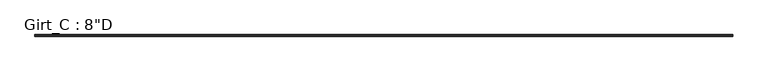
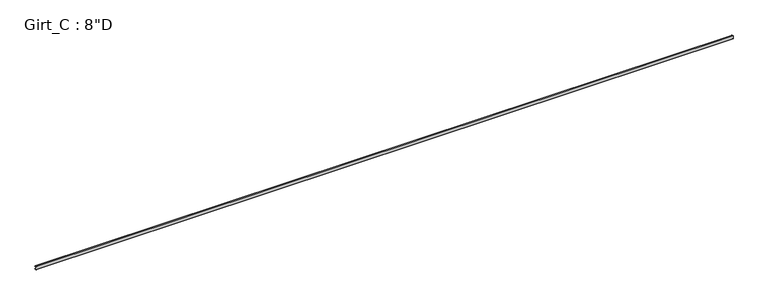
"""IFC4 building model written with IfcOpenShell, lengths in millimetres: beam geometry."""

import ifcopenshell
import ifcopenshell.guid

model = None  # the IFC model being written
_history = None  # IfcOwnerHistory: only IFC2X3 demands one
_inside = {}  # id of a spatial element -> (the spatial element, [elements in it])
_under = {}  # id of a project, library or spatial element -> (it, [spatial elements below it])
_declared = {}  # id of a project -> (the project, [libraries it declares])
_typed = {}  # id of a type object -> (the type object, [elements of that type])
_made_of = {}  # id of a material, layer set ... -> (it, [elements and type objects made of it])


def new_model(schema):
    """Start an empty IFC model of exactly this schema.

    Asked for "IFC4X3", IfcOpenShell would pick the latest addendum, in which some entities
    have other attributes; the version numbers below select the first issue.
    IFC2X3 requires an IfcOwnerHistory on every rooted entity: one is made here for all.
    """
    global model, _history
    if schema == "IFC4X3":
        model = ifcopenshell.file(schema_version=(4, 3, 0, 0))
    else:
        model = ifcopenshell.file(schema=schema)
    _inside.clear()
    _under.clear()
    _declared.clear()
    _typed.clear()
    _made_of.clear()
    _history = None
    if model.schema == "IFC2X3":
        org = make("IfcOrganization", Name="unknown")
        user = make(
            "IfcPersonAndOrganization",
            ThePerson=make("IfcPerson", FamilyName="unknown"),
            TheOrganization=org,
        )
        app = make(
            "IfcApplication",
            ApplicationDeveloper=org,
            Version="unknown",
            ApplicationFullName="unknown",
            ApplicationIdentifier="unknown",
        )
        _history = make(
            "IfcOwnerHistory",
            OwningUser=user,
            OwningApplication=app,
            ChangeAction="ADDED",
            CreationDate=0,
        )
    return model


def make(cls, **values):
    """One entity of the class cls with the attributes given. An attribute that is None is left unset."""
    return model.create_entity(
        cls, **{name: value for name, value in values.items() if value is not None}
    )


def rooted(cls, **values):
    """An entity with a GlobalId (a new one), such as an element, a storey or a relation."""
    return make(cls, GlobalId=ifcopenshell.guid.new(), OwnerHistory=_history, **values)


def si_unit(unit_type, name, prefix=None):
    """IfcSIUnit, for example si_unit("LENGTHUNIT", "METRE", prefix="MILLI")."""
    return make("IfcSIUnit", UnitType=unit_type, Prefix=prefix, Name=name)


def assignment(units):
    """IfcUnitAssignment: the units of a project."""
    return None if units is None else make("IfcUnitAssignment", Units=units)


def point(xyz):
    """IfcCartesianPoint."""
    return None if xyz is None else make("IfcCartesianPoint", Coordinates=xyz)


def direction(xyz):
    """IfcDirection."""
    return None if xyz is None else make("IfcDirection", DirectionRatios=xyz)


def frame(location, z_axis=None, x_axis=None):
    """IfcAxis2Placement3D, a coordinate frame: its origin and axes. An axis left out is left unset."""
    return make(
        "IfcAxis2Placement3D",
        Location=point(location),
        Axis=direction(z_axis),
        RefDirection=direction(x_axis),
    )


def frame_2d(location, x_axis=None):
    """IfcAxis2Placement2D, a coordinate frame in the plane: its origin and x axis."""
    return make(
        "IfcAxis2Placement2D", Location=point(location), RefDirection=direction(x_axis)
    )


def origin():
    """The frame at (0, 0, 0) with its axes left unset."""
    return frame((0.0, 0.0, 0.0))


def place(relative_to, where):
    """IfcLocalPlacement: puts the frame where relative to a parent placement (None: the world)."""
    return make(
        "IfcLocalPlacement", PlacementRelTo=relative_to, RelativePlacement=where
    )


def context(
    kind, dimensions, precision=None, world=None, true_north=None, identifier=None
):
    """IfcGeometricRepresentationContext, for example the 3D "Model" context."""
    return make(
        "IfcGeometricRepresentationContext",
        ContextIdentifier=identifier,
        ContextType=kind,
        CoordinateSpaceDimension=dimensions,
        Precision=precision,
        WorldCoordinateSystem=world,
        TrueNorth=true_north,
    )


def project(units=None, contexts=None):
    """IfcProject with its units and contexts."""
    return rooted(
        "IfcProject",
        Name="project",
        RepresentationContexts=contexts,
        UnitsInContext=assignment(units),
    )


def spatial(cls, under=None, at=None, **own):
    """A site, building, storey or space (cls), placed at a placement, below another one or the project."""
    s = rooted(cls, ObjectPlacement=at, **own)
    if under is not None:
        _under.setdefault(under.id(), (under, []))[1].append(s)
    return s


def polyline(points):
    """IfcPolyline through the points."""
    return make("IfcPolyline", Points=[point(p) for p in points])


def circle_curve(where, radius):
    """IfcCircle in the frame where."""
    return make("IfcCircle", Position=where, Radius=radius)


def trimmed(basis, trim1, trim2, sense, master):
    """IfcTrimmedCurve: the piece of a basis curve between two trims."""
    return make(
        "IfcTrimmedCurve",
        BasisCurve=basis,
        Trim1=trim1,
        Trim2=trim2,
        SenseAgreement=sense,
        MasterRepresentation=master,
    )


def segment(curve, same_sense, transition):
    """IfcCompositeCurveSegment."""
    return make(
        "IfcCompositeCurveSegment",
        Transition=transition,
        SameSense=same_sense,
        ParentCurve=curve,
    )


def composite_curve(segments, self_intersect=None):
    """IfcCompositeCurve: segments joined end to end."""
    return make("IfcCompositeCurve", Segments=segments, SelfIntersect=self_intersect)


def outline(outer, holes=None, kind="AREA"):
    """IfcArbitraryClosedProfileDef: a profile drawn as a closed curve; with holes, ...WithVoids."""
    if holes is None:
        return make("IfcArbitraryClosedProfileDef", ProfileType=kind, OuterCurve=outer)
    return make(
        "IfcArbitraryProfileDefWithVoids",
        ProfileType=kind,
        OuterCurve=outer,
        InnerCurves=holes,
    )


def extrude(swept, where, along, depth):
    """IfcExtrudedAreaSolid: the profile swept, set in the frame where, extruded along a direction by depth."""
    return make(
        "IfcExtrudedAreaSolid",
        SweptArea=swept,
        Position=where,
        ExtrudedDirection=direction(along),
        Depth=depth,
    )


def shape(context_of_items, identifier, shape_type, items):
    """IfcShapeRepresentation: the items that make up one representation, for example the "Body"."""
    return make(
        "IfcShapeRepresentation",
        ContextOfItems=context_of_items,
        RepresentationIdentifier=identifier,
        RepresentationType=shape_type,
        Items=items,
    )


def source(mapping_origin, context_of_items, identifier, shape_type, items):
    """IfcRepresentationMap: a shape defined once, which mapped items show again and again."""
    return make(
        "IfcRepresentationMap",
        MappingOrigin=mapping_origin,
        MappedRepresentation=shape(context_of_items, identifier, shape_type, items),
    )


def transform(
    local_origin,
    x_axis=None,
    y_axis=None,
    z_axis=None,
    scale=None,
    scale2=None,
    scale3=None,
    uniform=True,
):
    """IfcCartesianTransformationOperator3D, or its non-uniform kind. x_axis, y_axis, z_axis: its Axis1, 2, 3."""
    if uniform:
        return make(
            "IfcCartesianTransformationOperator3D",
            Axis1=direction(x_axis),
            Axis2=direction(y_axis),
            LocalOrigin=point(local_origin),
            Scale=scale,
            Axis3=direction(z_axis),
        )
    return make(
        "IfcCartesianTransformationOperator3DnonUniform",
        Axis1=direction(x_axis),
        Axis2=direction(y_axis),
        LocalOrigin=point(local_origin),
        Scale=scale,
        Axis3=direction(z_axis),
        Scale2=scale2,
        Scale3=scale3,
    )


def mapped(mapping_source, mapping_target):
    """IfcMappedItem: shows the shape of a source again, moved by a transform."""
    return make(
        "IfcMappedItem", MappingSource=mapping_source, MappingTarget=mapping_target
    )


def made_of(thing, what):
    """Note that an element or type object is made of a material, layer set ...; save() writes the relation."""
    if what is not None:
        _made_of.setdefault(what.id(), (what, []))[1].append(thing)
    return thing


def element(
    cls,
    number,
    at=None,
    inside=None,
    cuts=None,
    type_object=None,
    material=None,
    context=None,
    identifier="Body",
    shape_type=None,
    held_by="IfcProductDefinitionShape",
    body=None,
    shapes=None,
    **own,
):
    """One element of the class cls, such as IfcWall. Its Tag is "e" and its number.

    at: its placement. inside: the storey or other place that contains it. cuts: it is an
    opening in that element (IfcRelVoidsElement). A single representation is given by context,
    identifier, shape_type and body (its items); several are given by shapes. held_by: the class
    of the entity that holds the representations. save() writes the other relations.
    """
    e = rooted(cls, Tag="e%d" % number, ObjectPlacement=at, **own)
    if body is not None:
        shapes = [shape(context, identifier, shape_type, body)]
    if shapes is not None:
        e.Representation = make(held_by, Representations=shapes)
    if inside is not None:
        _inside.setdefault(inside.id(), (inside, []))[1].append(e)
    if cuts is not None:
        rooted(
            "IfcRelVoidsElement", RelatingBuildingElement=cuts, RelatedOpeningElement=e
        )
    if type_object is not None:
        _typed.setdefault(type_object.id(), (type_object, []))[1].append(e)
    return made_of(e, material)


def aggregate(whole, parts):
    """IfcRelAggregates: a whole, such as a stair, and the parts it consists of."""
    return rooted("IfcRelAggregates", RelatingObject=whole, RelatedObjects=parts)


def save(model, path):
    """Write the relations noted so far, then the file.

    IfcRelAggregates (storeys below a building ...), IfcRelContainedInSpatialStructure (elements
    in a storey), IfcRelDefinesByType, IfcRelAssociatesMaterial and IfcRelDeclares: one each for
    every whole, place, type object, material and project.
    """
    for whole, parts in _under.values():
        aggregate(whole, parts)
    for where, things in _inside.values():
        rooted(
            "IfcRelContainedInSpatialStructure",
            RelatedElements=things,
            RelatingStructure=where,
        )
    for kind, things in _typed.values():
        rooted("IfcRelDefinesByType", RelatedObjects=things, RelatingType=kind)
    for what, things in _made_of.values():
        rooted("IfcRelAssociatesMaterial", RelatedObjects=things, RelatingMaterial=what)
    for by, libraries in _declared.values():
        rooted("IfcRelDeclares", RelatingContext=by, RelatedDefinitions=libraries)
    model.write(path)


def beam_c287abb1(model_context):
    return source(origin(), model_context, "Body", "SweptSolid", [
        extrude(outline(composite_curve([segment(polyline([(87.5109375, 101.6), (99.7560415, 87.0068534), (97.6278742, 85.221109), (86.2154765, 98.821875), (3.3005807, 98.821875)]), True, "CONTINUOUS"), segment(trimmed(circle_curve(frame_2d((3.3741066, 96.8381931)), 1.9850441), [point((3.3005807, 98.821875))], [point((1.3890625, 96.8381931))], True, "CARTESIAN"), True, "CONTINUOUS"), segment(polyline([(1.3890625, 96.8381931), (1.3890625, -96.8389339)]), True, "CONTINUOUS"), segment(trimmed(circle_curve(frame_2d((3.3748024, -96.8389339)), 1.9857399), [point((1.3890625, -96.8389339))], [point((3.2694106, -98.821875))], True, "CARTESIAN"), True, "CONTINUOUS"), segment(polyline([(3.2694106, -98.821875), (86.2154765, -98.821875), (97.6510975, -85.1934327), (99.7792647, -86.979177), (87.5109375, -101.6), (3.3734375, -101.6)]), True, "CONTINUOUS"), segment(trimmed(circle_curve(frame_2d((3.3734375, -96.8375)), 4.7625), [point((3.3734375, -101.6))], [point((-1.3890625, -96.8375))], False, "CARTESIAN"), True, "CONTINUOUS"), segment(polyline([(-1.3890625, -96.8375), (-1.3890625, 96.8375)]), True, "CONTINUOUS"), segment(trimmed(circle_curve(frame_2d((3.3734375, 96.8375)), 4.7625), [point((-1.3890625, 96.8375))], [point((3.3734375, 101.6))], False, "CARTESIAN"), True, "CONTINUOUS"), segment(polyline([(3.3734375, 101.6), (87.5109375, 101.6)]), True, "CONTINUOUS")], self_intersect=False)), frame((-21958.3, 0.0, 0.0), z_axis=(1.0, 0.0, 0.0), x_axis=(0.0, 1.0, 0.0)), (0.0, 0.0, 1.0), 43891.2),
    ])


if __name__ == "__main__":
    model = new_model("IFC4")
    model_context = context("Model", 3, world=origin())
    ifc_project = project(units=[si_unit("LENGTHUNIT", "METRE", prefix="MILLI")], contexts=[model_context])
    site = spatial("IfcSite", under=ifc_project)
    building = spatial("IfcBuilding", under=site)
    placement = place(None, origin())
    beam_shape = beam_c287abb1(model_context)
    element("IfcBeam", 1, ObjectType="Girt_C : 8\"D", at=placement, inside=building, context=model_context, shape_type="MappedRepresentation", body=[
        mapped(beam_shape, transform((0.0, 0.0, 0.0), x_axis=(1.0, 0.0, 0.0), y_axis=(0.0, 1.0, 0.0), z_axis=(0.0, 0.0, 1.0))),
    ])
    save(model, "model.ifc")

# Revit data of these elements
# Type "Girt_C : 8\"D"
#   half leg = 0' - 1 3/4"
#   Web_Thickness = 0' - 0 7/64"
#   Length [instance default] = 10' - 0"
#   Leg_1 = 0' - 3 1/2"
#   Height = 0' - 8"
#   Structural Material [instance default] = none
# Element 1 (IfcBeam, "Girt_C : 8\"D")
#   Structural Material = CEE' SECTION (8.0x3.5C - SEE STRUCT. DWGS)
#   Materials on its faces: "CEE' SECTION (8.0x3.5C - SEE STRUCT. DWGS)"
# Materials
#   "CEE' SECTION (8.0x3.5C - SEE STRUCT. DWGS)": class "Metal", colour RGB 137 146 153, transparency 0, Description = "Steel, mill finish", Cost = 0
